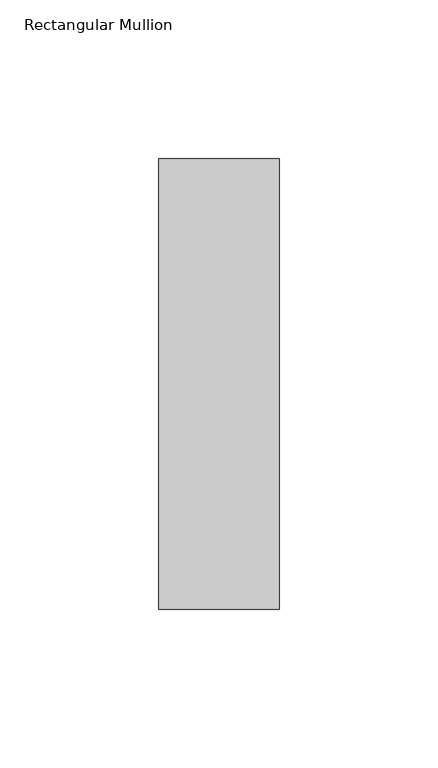
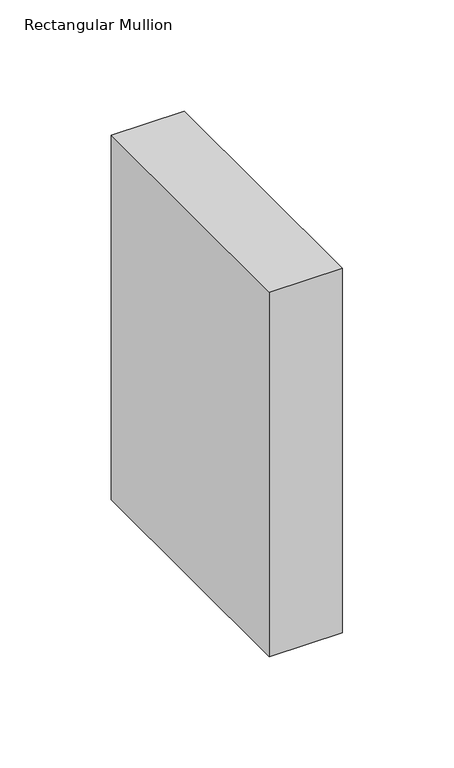
"""IFC4 building model written with IfcOpenShell, lengths in millimetres: member geometry, Rectangular Mullion : NLRS_21_CWM_hsb-regel 38x142_gen_rsf."""

from ifc_helpers import new_model, si_unit, frame, origin, place, context, project, spatial, polyline, outline, extrude, source, transform, mapped, element, save


def rectangular_mullion_fa24708d(model_context):
    return source(origin(), model_context, "Body", "SweptSolid", [
        extrude(outline(polyline([(0.0, -71.0), (-38.0, -71.0), (-38.0, 71.0), (0.0, 71.0), (0.0, -71.0)])), frame((0.0, 0.0, -199.9999997), z_axis=(0.0, 0.0, 1.0), x_axis=(1.0, 0.0, 0.0)), (0.0, 0.0, 1.0), 199.9999997),
    ])


if __name__ == "__main__":
    model = new_model("IFC4")
    model_context = context("Model", 3, world=origin())
    ifc_project = project(units=[si_unit("LENGTHUNIT", "METRE", prefix="MILLI")], contexts=[model_context])
    site = spatial("IfcSite", under=ifc_project)
    building = spatial("IfcBuilding", under=site)
    placement = place(None, origin())
    rectangular_mullion_shape = rectangular_mullion_fa24708d(model_context)
    element("IfcMember", 1, ObjectType="Rectangular Mullion : NLRS_21_CWM_hsb-regel 38x142_gen_rsf", at=placement, inside=building, context=model_context, shape_type="MappedRepresentation", body=[
        mapped(rectangular_mullion_shape, transform((0.0, 0.0, 0.0), x_axis=(1.0, 0.0, 0.0), y_axis=(0.0, 1.0, 0.0), z_axis=(0.0, 0.0, 1.0))),
    ])
    save(model, "model.ifc")

# Revit data of these elements
# Type "Rectangular Mullion : NLRS_21_CWM_hsb-regel 38x142_gen_rsf"
#   Export Type to IFC As = "IfcWall"
#   Type IfcGUID = "07M7mRoiH1CR8m_RSKIwpF"
#   Assembly Code = "21.10"
#   built-in parameter 1007322 = 0.465879 (stored number, unit not read)
#   built-in parameter 1007321 = 0.062336 (stored number, unit not read)
#   built-in parameter 1007320 = 0.062336 (stored number, unit not read)
# Element 1 (IfcMember, "Rectangular Mullion : NLRS_21_CWM_hsb-regel 38x142_gen_rsf")
#   Materials on its faces: "NLRS_i2_hout naaldhout vuren_gen_rsf"
# Materials
#   "NLRS_i2_hout naaldhout vuren_gen_rsf": class "I - Hout", colour RGB 234 199 147, transparency 0, Keynote = "i2", Manufacturer = "Revit Standards Foundation", URL = "www.revitstandards.org", Description = "hout vuren", Cost = 0
